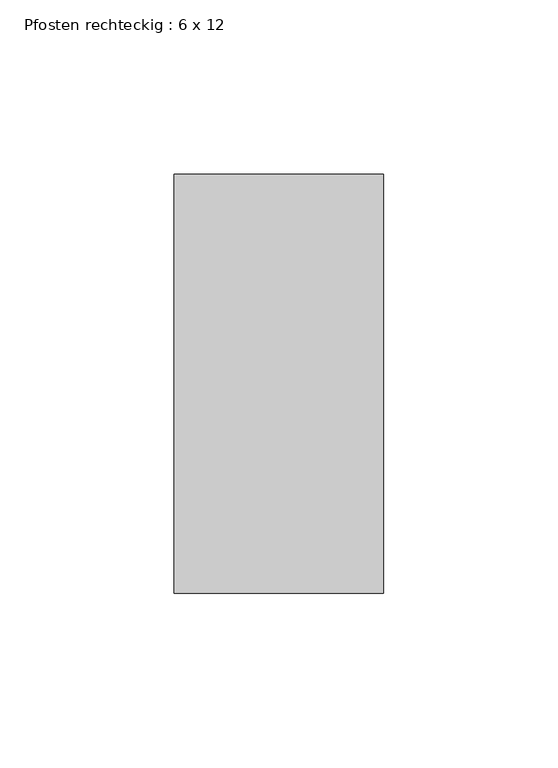
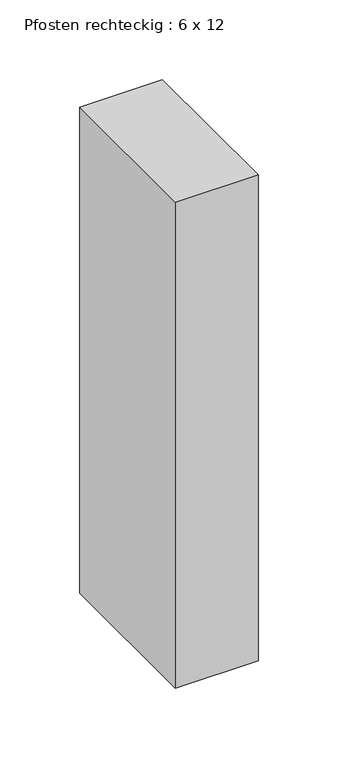
"""IFC4 building model written with IfcOpenShell, lengths in millimetres: member geometry, Pfosten rechteckig : 6 x 12."""

from ifc_helpers import new_model, si_unit, frame, origin, place, context, project, spatial, polyline, outline, extrude, source, transform, mapped, element, save


def pfosten_rechteckig_6_x_12_f461bf22(model_context):
    return source(origin(), model_context, "Body", "SweptSolid", [
        extrude(outline(polyline([(30.0, 60.0), (30.0, -60.0), (-30.0, -60.0), (-30.0, 60.0), (30.0, 60.0)])), frame((0.0, 0.0, -372.4999997), z_axis=(0.0, 0.0, 1.0), x_axis=(1.0, 0.0, 0.0)), (0.0, 0.0, 1.0), 372.4999997),
    ])


if __name__ == "__main__":
    model = new_model("IFC4")
    model_context = context("Model", 3, world=origin())
    ifc_project = project(units=[si_unit("LENGTHUNIT", "METRE", prefix="MILLI")], contexts=[model_context])
    site = spatial("IfcSite", under=ifc_project)
    building = spatial("IfcBuilding", under=site)
    placement = place(None, origin())
    pfosten_rechteckig_6_x_12_shape = pfosten_rechteckig_6_x_12_f461bf22(model_context)
    element("IfcMember", 1, ObjectType="Pfosten rechteckig : 6 x 12", at=placement, inside=building, context=model_context, shape_type="MappedRepresentation", body=[
        mapped(pfosten_rechteckig_6_x_12_shape, transform((0.0, 0.0, 0.0), x_axis=(1.0, 0.0, 0.0), y_axis=(0.0, 1.0, 0.0), z_axis=(0.0, 0.0, 1.0))),
    ])
    save(model, "model.ifc")

# Revit data of these elements
# Type "Pfosten rechteckig : 6 x 12"
#   built-in parameter 1007304 = 0.393701 (stored number, unit not read)
#   built-in parameter 1007301 = 0.0984252 (stored number, unit not read)
#   built-in parameter 1007300 = 0.0984252 (stored number, unit not read)
# Element 1 (IfcMember, "Pfosten rechteckig : 6 x 12")
#   Materials on its faces: "Metall - verzinkt"
# Materials
#   "Metall - verzinkt": class "Allgemeines", colour RGB 200 200 200, transparency 0, Cost = 0
